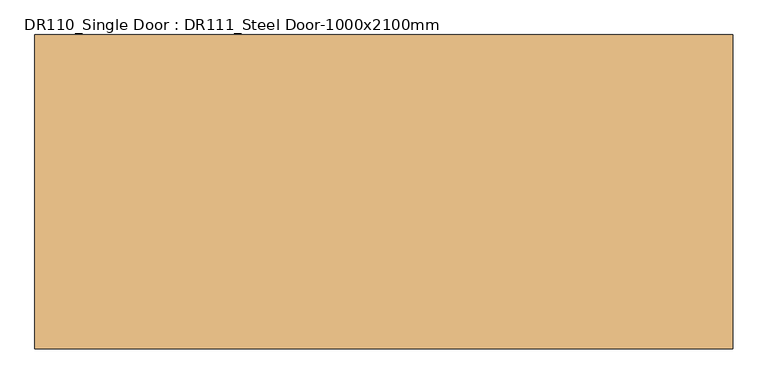
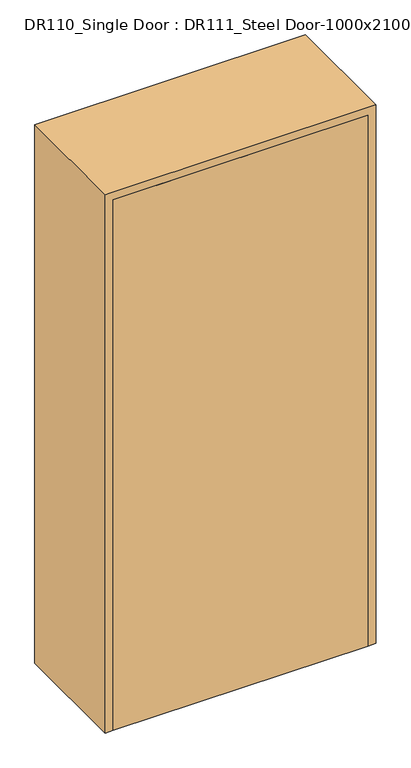
"""IFC4 building model written with IfcOpenShell, lengths in millimetres: door geometry, DR110_Single Door : DR111_Steel Door-1000x2100mm."""

from ifc_helpers import new_model, si_unit, origin, origin_with_axes, place, context, project, spatial, polyline, outline, extrude, faceted_brep, source, transform, mapped, element, save


def dr110_single_door_dr111_steel_door_1000x2100mm_3adf1b50(model_context):
    return source(origin(), model_context, "Body", "SolidModel", [
        extrude(outline(polyline([(470.0, -225.0), (-470.0, -225.0), (-470.0, -190.0), (470.0, -190.0), (470.0, -225.0)])), origin_with_axes(), (0.0, 0.0, 1.0), 2070.0),
        faceted_brep([(470.0, -225.0, 0.0), (470.0, -190.0, 0.0), (450.0, -190.0, 0.0), (450.0, 190.0, 0.0), (470.0, 190.0, 0.0), (470.0, 225.0, 0.0), (500.0, 225.0, 0.0), (500.0, -225.0, 0.0), (500.0, -225.0, 2100.0), (-500.0, -225.0, 2100.0), (-500.0, -225.0, 0.0), (-470.0, -225.0, 0.0), (-470.0, -225.0, 2070.0), (470.0, -225.0, 2070.0), (500.0, 225.0, 2100.0), (470.0, 225.0, 2070.0), (-470.0, 225.0, 2070.0), (-470.0, 225.0, 0.0), (-500.0, 225.0, 0.0), (-500.0, 225.0, 2100.0), (470.0, 190.0, 2070.0), (450.0, 190.0, 2050.0), (-450.0, 190.0, 2050.0), (-450.0, 190.0, 0.0), (-470.0, 190.0, 0.0), (-470.0, 190.0, 2070.0), (450.0, -190.0, 2050.0), (470.0, -190.0, 2070.0), (-470.0, -190.0, 2070.0), (-470.0, -190.0, 0.0), (-450.0, -190.0, 0.0), (-450.0, -190.0, 2050.0)], [[[0, 1, 2, 3, 4, 5, 6, 7]], [[7, 8, 9, 10, 11, 12, 13, 0]], [[6, 14, 8, 7]], [[5, 15, 16, 17, 18, 19, 14, 6]], [[4, 20, 15, 5]], [[3, 21, 22, 23, 24, 25, 20, 4]], [[2, 26, 21, 3]], [[1, 27, 28, 29, 30, 31, 26, 2]], [[0, 13, 27, 1]], [[12, 11, 29, 28]], [[11, 10, 18, 17, 24, 23, 30, 29]], [[19, 18, 10, 9]], [[25, 24, 17, 16]], [[31, 30, 23, 22]], [[14, 19, 9, 8]], [[20, 25, 16, 15]], [[26, 31, 22, 21]], [[13, 12, 28, 27]]]),
    ])


if __name__ == "__main__":
    model = new_model("IFC4")
    model_context = context("Model", 3, world=origin())
    ifc_project = project(units=[si_unit("LENGTHUNIT", "METRE", prefix="MILLI")], contexts=[model_context])
    site = spatial("IfcSite", under=ifc_project)
    building = spatial("IfcBuilding", under=site)
    placement = place(None, origin())
    dr110_single_door_dr111_steel_door_1000x2100mm_shape = dr110_single_door_dr111_steel_door_1000x2100mm_3adf1b50(model_context)
    element("IfcDoor", 1, ObjectType="DR110_Single Door : DR111_Steel Door-1000x2100mm", at=placement, inside=building, context=model_context, shape_type="MappedRepresentation", body=[
        mapped(dr110_single_door_dr111_steel_door_1000x2100mm_shape, transform((0.0, 0.0, 0.0), x_axis=(1.0, 0.0, 0.0), y_axis=(0.0, 1.0, 0.0), z_axis=(0.0, 0.0, 1.0))),
    ])
    save(model, "model.ifc")

# Revit data of these elements
# Type "DR110_Single Door : DR111_Steel Door-1000x2100mm"
#   Type Mark = "SD"
#   Analytic Construction = "<None>"
#   프레임 투영 외부. = 25 mm
#   프레임 투영 내부. = 25 mm
#   프레임 폭 = 75 mm
#   Height = 2100 mm
#   Width = 1000 mm
#   Define Thermal Properties by = 1
#   문 패널 = SD1 문 패널
#   문 프레임 = A04AQ098-00002_Steel Door_non FP_single
#   Function = (empty or 0)
#   Wall Closure = (empty or 0)
# Element 1 (IfcDoor, "DR110_Single Door : DR111_Steel Door-1000x2100mm")
#   Materials on its faces: "A04AQ098-00002_Steel Door_non FP_single", "SD1 문 패널"
# Materials
#   "SD1 문 패널": class "금속", colour RGB 247 247 247, transparency 0, Description = "STEEL DOOR (1000Wx2100H)"
#   "A04AQ098-00002_Steel Door_non FP_single": class "금속", colour RGB 247 247 247, transparency 0, Description = "Steel Door", W00) Work Master Code = "A04AQ098-00002", W01) Work Master_Lv1 = "Finishing Work", W02) Work Master_Lv2 = "Door & Window Work", W03) Work Master_Spec.1 = "Steel Door w/ Steel Frame", W04) Work Master_Spec.2 = "Fire Protective Rating: N/A, Single Door", W05) Work Master_Spec.3 = "w/ Hardware & Accessories", Cost = 0
